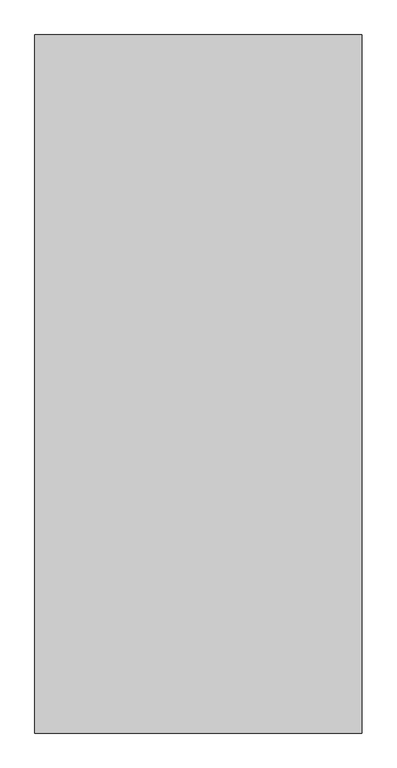
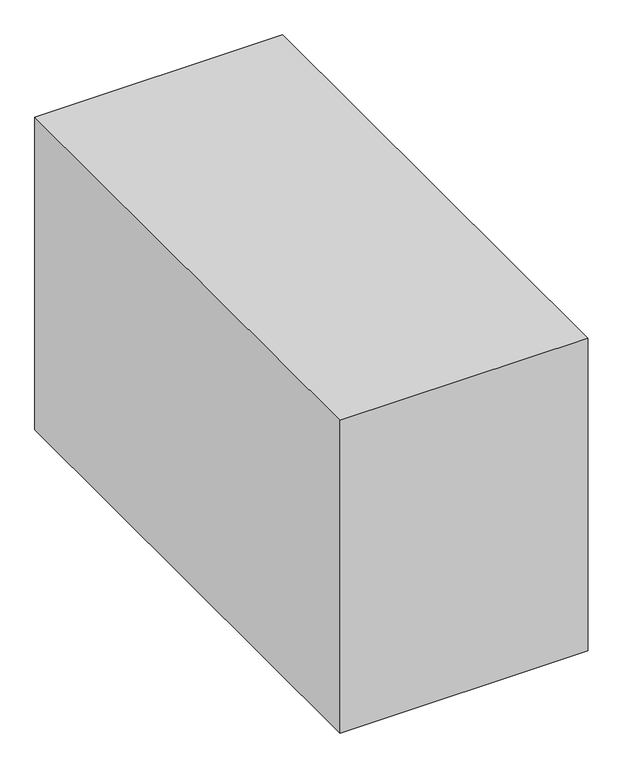
"""IFC4 building model written with IfcOpenShell, lengths in millimetres: proxy geometry, Space Planning Box_hec : Space Planning Box_hec."""

from ifc_helpers import new_model, si_unit, origin, origin_with_axes, place, context, project, spatial, polyline, outline, extrude, source, transform, mapped, element, save


def generic_models_96097b63(model_context):
    return source(origin(), model_context, "Body", "SweptSolid", [
        extrude(outline(polyline([(2250.0, 4800.0), (2250.0, -4800.0), (-2250.0, -4800.0), (-2250.0, 4800.0), (2250.0, 4800.0)])), origin_with_axes(), (0.0, 0.0, 1.0), 6000.0),
    ])


if __name__ == "__main__":
    model = new_model("IFC4")
    model_context = context("Model", 3, world=origin())
    ifc_project = project(units=[si_unit("LENGTHUNIT", "METRE", prefix="MILLI")], contexts=[model_context])
    site = spatial("IfcSite", under=ifc_project)
    building = spatial("IfcBuilding", under=site)
    placement = place(None, origin())
    generic_models_shape = generic_models_96097b63(model_context)
    element("IfcBuildingElementProxy", 1, Name="Space Planning Box_hec : Space Planning Box_hec", ObjectType="Space Planning Box_hec : Space Planning Box_hec", at=placement, inside=building, context=model_context, shape_type="MappedRepresentation", body=[
        mapped(generic_models_shape, transform((0.0, 0.0, 0.0), x_axis=(1.0, 0.0, 0.0), y_axis=(0.0, 1.0, 0.0), z_axis=(0.0, 0.0, 1.0))),
    ])
    save(model, "model.ifc")

# Revit data of these elements
# Type "Space Planning Box_hec : Space Planning Box_hec"
#   Type Comments = "..."
#   Room Name [instance default] = "?"
#   Interior Finish [instance default] = ""
#   Exterior Finish [instance default] = ""
#   Department [instance default] = ""
#   Assembly Code = "..."
#   Width [instance default] = 1524 mm
#   Program Area [instance default] = 0.00 m²
#   Length [instance default] = 1524 mm
#   Height [instance default] = 1524 mm
#   Area [instance default] = 2.32258 m²
#   Fill Color [instance default] = Cyan
#   Default Elevation = 0
# Element 1 (IfcBuildingElementProxy, "Space Planning Box_hec : Space Planning Box_hec")
#   Room Name = "Shift Office Room"
#   Interior Finish = "IF2-1"
#   Exterior Finish = "EF1"
#   Department = "AR"
#   Width = 4500 mm
#   Program Area = 43.20 m²
#   Length = 9600 mm
#   Height = 6000 mm
#   Area = 43.20 m²
#   Fill Color = Lavender
#   Materials on its faces: "Lavender"
# Materials
#   "Cyan": class "Generic", colour RGB 0 255 255, transparency 0.2, Cost = 0
#   "Lavender": class "Generic", colour RGB 186 85 211, transparency 0.2, Cost = 0
